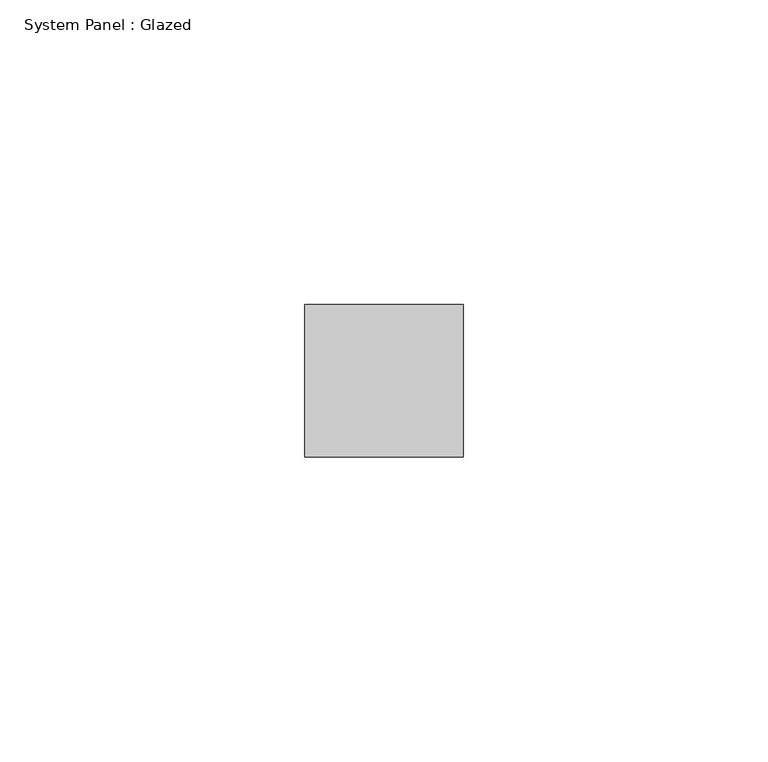
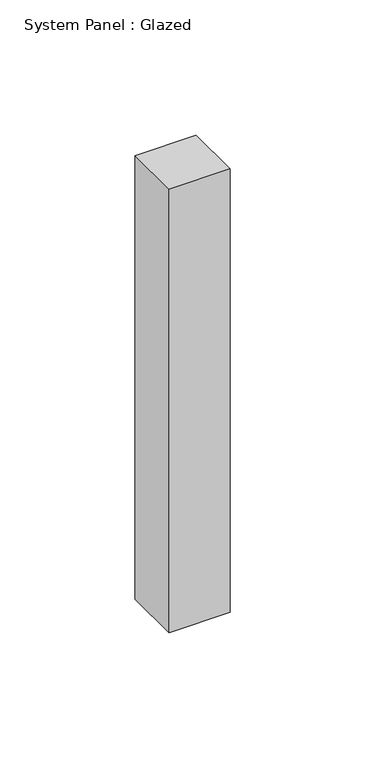
"""IFC4 building model written with IfcOpenShell, lengths in millimetres: plate geometry, System Panel : Glazed."""

from ifc_helpers import new_model, si_unit, origin, origin_with_axes, place, context, project, spatial, polyline, outline, extrude, source, transform, mapped, element, save


def system_panel_glazed_b8c9dfa1(model_context):
    return source(origin(), model_context, "Body", "SweptSolid", [
        extrude(outline(polyline([(12.980414, 24.5), (-12.980414, 24.5), (-12.980414, 49.5), (12.980414, 49.5), (12.980414, 24.5)])), origin_with_axes(), (0.0, 0.0, 1.0), 200.0),
    ])


if __name__ == "__main__":
    model = new_model("IFC4")
    model_context = context("Model", 3, world=origin())
    ifc_project = project(units=[si_unit("LENGTHUNIT", "METRE", prefix="MILLI")], contexts=[model_context])
    site = spatial("IfcSite", under=ifc_project)
    building = spatial("IfcBuilding", under=site)
    placement = place(None, origin())
    system_panel_glazed_shape = system_panel_glazed_b8c9dfa1(model_context)
    element("IfcPlate", 1, ObjectType="System Panel : Glazed", at=placement, inside=building, context=model_context, shape_type="MappedRepresentation", body=[
        mapped(system_panel_glazed_shape, transform((0.0, 0.0, 0.0), x_axis=(1.0, 0.0, 0.0), y_axis=(0.0, 1.0, 0.0), z_axis=(0.0, 0.0, 1.0))),
    ])
    save(model, "model.ifc")

# Revit data of these elements
# Element 1 (IfcPlate, "System Panel : Glazed")
#   Materials on its faces: "Glass"
# Materials
#   "Glass": class "Glass", colour RGB 218 227 224, transparency 0.85, Description = "Soda Lime Glass", Cost = 0
